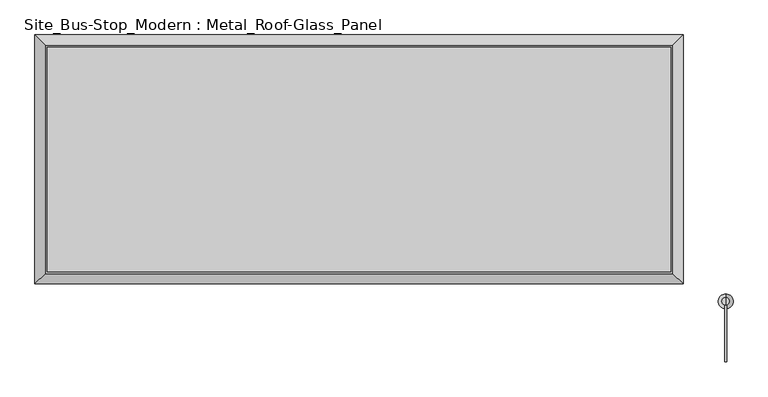
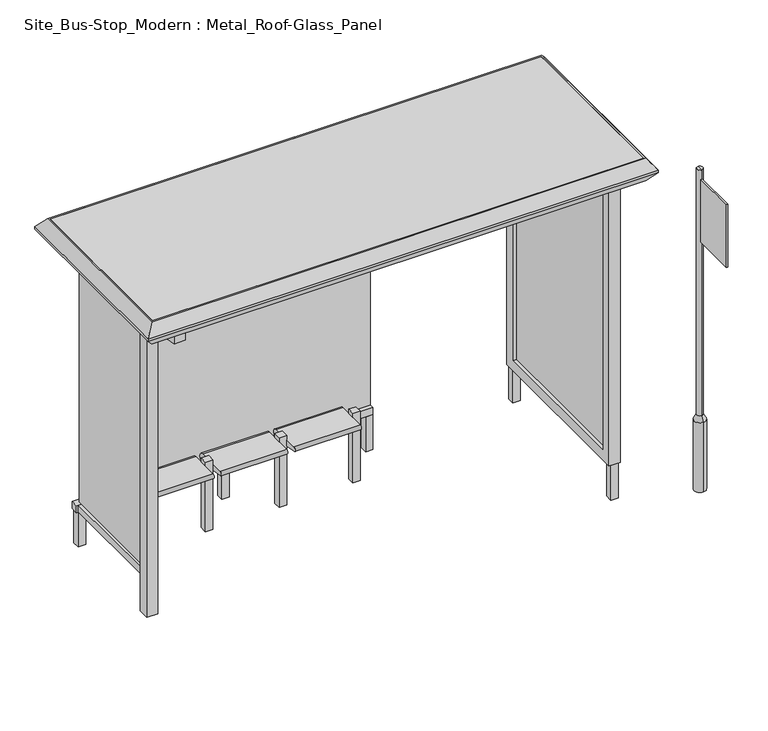
"""IFC4 building model written with IfcOpenShell, lengths in millimetres: geographic element geometry, Site_Bus-Stop_Modern : Metal_Roof-Glass_Panel."""

from ifc_helpers import new_model, si_unit, point, frame, frame_2d, origin, origin_with_axes, place, context, project, spatial, polyline, circle_curve, trimmed, segment, composite_curve, outline, extrude, faceted_brep, source, transform, mapped, element, save
from ifc_brep_helpers import plane_surface, cylinder_surface, revolved_surface, advanced_brep


def site_bus_stop_modern_metal_roof_glass_panel_3fdf870d(model_context):
    return source(origin(), model_context, "Body", "SolidModel", [
        extrude(outline(polyline([(1957.5, -1680.3732439), (1957.5, -1380.3732439), (1967.5, -1380.3732439), (1967.5, -1680.3732439), (1957.5, -1680.3732439)])), frame((0.0, 0.0, 1784.6), z_axis=(0.0, 0.0, 1.0), x_axis=(1.0, 0.0, 0.0)), (0.0, 0.0, 1.0), 450.0),
        advanced_brep(
        [(1962.5, -1398.2604073, 500.0), (1962.5, -1318.2604073, 500.0), (1962.5, -1318.2604073, 0.0), (1962.5, -1398.2604073, 0.0), (1962.5, -1378.2604073, 534.6), (1962.5, -1338.2604073, 534.6), (1962.5, -1378.2604073, 2300.0), (1962.5, -1338.2604073, 2300.0), (1962.5, -1358.2604073, 2300.0), (1962.5, -1358.2604073, 0.0)],
        [
            (0, 1, circle_curve(frame((1962.5, -1358.2604073, 500.0), z_axis=(0.0, 0.0, -1.0), x_axis=(0.0, 1.0, 0.0)), 40.0)),
            (1, 2),
            (2, 3, circle_curve(frame((1962.5, -1358.2604073, 0.0), z_axis=(0.0, 0.0, 1.0), x_axis=(0.0, 1.0, 0.0)), 40.0)),
            (3, 0),
            (1, 0, circle_curve(frame((1962.5, -1358.2604073, 500.0), z_axis=(0.0, 0.0, -1.0), x_axis=(0.0, 1.0, 0.0)), 40.0)),
            (3, 2, circle_curve(frame((1962.5, -1358.2604073, 0.0), z_axis=(0.0, 0.0, 1.0), x_axis=(0.0, 1.0, 0.0)), 40.0)),
            (4, 5, circle_curve(frame((1962.5, -1358.2604073, 534.6), z_axis=(0.0, 0.0, -1.0), x_axis=(0.0, 1.0, 0.0)), 20.0)),
            (5, 1),
            (0, 4),
            (5, 4, circle_curve(frame((1962.5, -1358.2604073, 534.6), z_axis=(0.0, 0.0, -1.0), x_axis=(0.0, 1.0, 0.0)), 20.0)),
            (6, 7, circle_curve(frame((1962.5, -1358.2604073, 2300.0), z_axis=(0.0, 0.0, -1.0), x_axis=(0.0, 1.0, 0.0)), 20.0)),
            (7, 5),
            (4, 6),
            (7, 6, circle_curve(frame((1962.5, -1358.2604073, 2300.0), z_axis=(0.0, 0.0, -1.0), x_axis=(0.0, 1.0, 0.0)), 20.0)),
            (8, 7),
            (6, 8),
            (2, 9),
            (9, 3),
        ],
        [
            cylinder_surface(frame((1962.5, -1358.2604073, -120.0), z_axis=(0.0, 0.0, 1.0), x_axis=(0.0, 1.0, 0.0)), 40.0),
            revolved_surface(polyline([(1962.5, -1318.2604073, 500.0), (1962.5, -1338.2604073, 534.6)]), (1962.5, -1358.2604073, -120.0), (0.0, 0.0, 1.0)),
            cylinder_surface(frame((1962.5, -1358.2604073, -120.0), z_axis=(0.0, 0.0, 1.0), x_axis=(0.0, 1.0, 0.0)), 20.0),
            plane_surface(frame((1962.5, -1358.2604073, 2300.0), z_axis=(0.0, 0.0, 1.0), x_axis=(0.0, 1.0, 0.0))),
            plane_surface(frame((1962.5, -1358.2604073, 0.0), z_axis=(0.0, 0.0, -1.0), x_axis=(0.0, 1.0, 0.0))),
        ],
        [
            (0, [[1, 2, 3, 4]]),
            (0, [[5, -4, 6, -2]]),
            (1, [[7, 8, -1, 9]]),
            (1, [[10, -9, -5, -8]]),
            (2, [[11, 12, -7, 13]]),
            (2, [[14, -13, -10, -12]]),
            (3, [[15, -11, 16]]),
            (3, [[-16, -14, -15]]),
            (4, [[-3, 17, 18]]),
            (4, [[-6, -18, -17]]),
        ],
    ),
        faceted_brep([(1735.0, 65.0, 2310.0), (1680.0, 10.0, 2380.0), (1680.0, -1210.0, 2380.0), (1735.0, -1265.0, 2310.0), (1735.0, 65.0, 2290.0), (1735.0, -1265.0, 2290.0), (1680.0, 10.0, 2220.0), (1680.0, -1210.0, 2220.0), (1670.0, 0.0, 2380.0), (1670.0, 0.0, 2220.0), (1670.0, -1200.0, 2220.0), (1670.0, -1200.0, 2380.0), (-1672.5, -1210.0, 2380.0), (-1727.5, -1265.0, 2310.0), (-1727.5, -1265.0, 2290.0), (-1672.5, -1210.0, 2220.0), (-1662.5, -1200.0, 2220.0), (-1662.5, -1200.0, 2380.0), (-1672.5, 10.0, 2380.0), (-1727.5, 65.0, 2310.0), (-1727.5, 65.0, 2290.0), (-1672.5, 10.0, 2220.0), (-1662.5, 0.0, 2220.0), (-1662.5, 0.0, 2380.0)], [[[0, 1, 2, 3]], [[4, 0, 3, 5]], [[6, 4, 5, 7]], [[8, 9, 10, 11]], [[3, 2, 12, 13]], [[5, 3, 13, 14]], [[7, 5, 14, 15]], [[11, 10, 16, 17]], [[13, 12, 18, 19]], [[14, 13, 19, 20]], [[15, 14, 20, 21]], [[17, 16, 22, 23]], [[19, 18, 1, 0]], [[20, 19, 0, 4]], [[21, 20, 4, 6]], [[7, 15, 21, 6], [9, 22, 16, 10]], [[23, 22, 9, 8]], [[1, 18, 12, 2], [11, 17, 23, 8]]]),
        extrude(outline(polyline([(-1662.5, -1200.0), (-1662.5, 0.0), (1670.0, 0.0), (1670.0, -1200.0), (-1662.5, -1200.0)])), frame((0.0, 0.0, 2220.0), z_axis=(0.0, 0.0, 1.0), x_axis=(1.0, 0.0, 0.0)), (0.0, 0.0, 1.0), 160.0),
        extrude(outline(polyline([(1490.0, -50.0), (1490.0, -1150.0), (1480.0, -1150.0), (1480.0, -50.0), (1490.0, -50.0)])), frame((0.0, 0.0, 300.0), z_axis=(0.0, 0.0, 1.0), x_axis=(1.0, 0.0, 0.0)), (0.0, 0.0, 1.0), 1870.0),
        extrude(outline(polyline([(1460.0, -1150.0), (1460.0, -50.0), (1470.0, -50.0), (1470.0, -1150.0), (1460.0, -1150.0)])), frame((0.0, 0.0, 300.0), z_axis=(0.0, 0.0, 1.0), x_axis=(1.0, 0.0, 0.0)), (0.0, 0.0, 1.0), 1870.0),
        faceted_brep([(1512.5, 0.0, 250.0), (1437.5, 0.0, 250.0), (1437.5, 0.0, 2220.0), (1512.5, 0.0, 2220.0), (1487.5, -75.0, 325.0), (1512.5, -75.0, 325.0), (1512.5, -75.0, 2145.0), (1487.5, -75.0, 2145.0), (1462.5, -50.0, 300.0), (1487.5, -50.0, 300.0), (1487.5, -50.0, 2170.0), (1462.5, -50.0, 2170.0), (1437.5, -75.0, 325.0), (1462.5, -75.0, 325.0), (1462.5, -75.0, 2145.0), (1437.5, -75.0, 2145.0), (1437.5, -1200.0, 2220.0), (1512.5, -1200.0, 2220.0), (1512.5, -1125.0, 2145.0), (1487.5, -1125.0, 2145.0), (1487.5, -1150.0, 2170.0), (1462.5, -1150.0, 2170.0), (1462.5, -1125.0, 2145.0), (1437.5, -1125.0, 2145.0), (1437.5, -1200.0, 250.0), (1512.5, -1200.0, 250.0), (1512.5, -1125.0, 325.0), (1487.5, -1125.0, 325.0), (1487.5, -1150.0, 300.0), (1462.5, -1150.0, 300.0), (1462.5, -1125.0, 325.0), (1437.5, -1125.0, 325.0)], [[[0, 1, 2, 3]], [[4, 5, 6, 7]], [[8, 9, 10, 11]], [[12, 13, 14, 15]], [[3, 2, 16, 17]], [[7, 6, 18, 19]], [[11, 10, 20, 21]], [[15, 14, 22, 23]], [[17, 16, 24, 25]], [[19, 18, 26, 27]], [[21, 20, 28, 29]], [[23, 22, 30, 31]], [[25, 24, 1, 0]], [[3, 17, 25, 0], [5, 26, 18, 6]], [[27, 26, 5, 4]], [[9, 28, 20, 10], [7, 19, 27, 4]], [[29, 28, 9, 8]], [[11, 21, 29, 8], [13, 30, 22, 14]], [[31, 30, 13, 12]], [[1, 24, 16, 2], [15, 23, 31, 12]]]),
        extrude(outline(polyline([(500.0, -20.0), (-1470.0, -20.0), (-1470.0, -10.0), (500.0, -10.0), (500.0, -20.0)])), frame((0.0, 0.0, 300.0), z_axis=(0.0, 0.0, 1.0), x_axis=(1.0, 0.0, 0.0)), (0.0, 0.0, 1.0), 1920.0),
        extrude(outline(polyline([(-800.0, 300.0), (-800.0, 2100.0), (-25.0, 2158.125), (-25.0, 300.0), (-800.0, 300.0)])), frame((-1480.0, 0.0, 0.0), z_axis=(1.0, 0.0, 0.0), x_axis=(0.0, 1.0, 0.0)), (0.0, 0.0, 1.0), 10.0),
        extrude(outline(composite_curve([segment(trimmed(circle_curve(frame_2d((-171.5367578, 436.9988667)), 33.0011333), [point((-171.5367578, 470.0))], [point((-171.5367578, 403.9977334))], False, "CARTESIAN"), True, "CONTINUOUS"), segment(polyline([(-171.5367578, 403.9977334), (-376.5367578, 440.1447644)]), True, "CONTINUOUS"), segment(trimmed(circle_curve(frame_2d((-376.5367578, 455.0723822)), 14.9276178), [point((-376.5367578, 440.1447644))], [point((-376.5367578, 470.0))], False, "CARTESIAN"), True, "CONTINUOUS"), segment(polyline([(-376.5367578, 470.0), (-171.5367578, 470.0)]), True, "CONTINUOUS")], self_intersect=False)), frame((-225.0, 0.0, 0.0), z_axis=(1.0, 0.0, 0.0), x_axis=(0.0, 1.0, 0.0)), (0.0, 0.0, 1.0), 450.0),
        extrude(outline(composite_curve([segment(trimmed(circle_curve(frame_2d((-171.5367578, 436.9988667)), 33.0011333), [point((-171.5367578, 470.0))], [point((-171.5367578, 403.9977334))], False, "CARTESIAN"), True, "CONTINUOUS"), segment(polyline([(-171.5367578, 403.9977334), (-376.5367578, 440.1447644)]), True, "CONTINUOUS"), segment(trimmed(circle_curve(frame_2d((-376.5367578, 455.0723822)), 14.9276178), [point((-376.5367578, 440.1447644))], [point((-376.5367578, 470.0))], False, "CARTESIAN"), True, "CONTINUOUS"), segment(polyline([(-376.5367578, 470.0), (-171.5367578, 470.0)]), True, "CONTINUOUS")], self_intersect=False)), frame((-725.0, 0.0, 0.0), z_axis=(1.0, 0.0, 0.0), x_axis=(0.0, 1.0, 0.0)), (0.0, 0.0, 1.0), 450.0),
        extrude(outline(composite_curve([segment(trimmed(circle_curve(frame_2d((-173.0011333, 436.9988667)), 33.0011333), [point((-173.0011333, 470.0))], [point((-173.0011333, 403.9977334))], False, "CARTESIAN"), True, "CONTINUOUS"), segment(polyline([(-173.0011333, 403.9977334), (-378.0011333, 440.1447644)]), True, "CONTINUOUS"), segment(trimmed(circle_curve(frame_2d((-378.0011333, 455.0723822)), 14.9276178), [point((-378.0011333, 440.1447644))], [point((-378.0011333, 470.0))], False, "CARTESIAN"), True, "CONTINUOUS"), segment(polyline([(-378.0011333, 470.0), (-173.0011333, 470.0)]), True, "CONTINUOUS")], self_intersect=False)), frame((-1225.0, 0.0, 0.0), z_axis=(1.0, 0.0, 0.0), x_axis=(0.0, 1.0, 0.0)), (0.0, 0.0, 1.0), 450.0),
        extrude(outline(polyline([(-1200.0, 2220.0), (0.0, 2220.0), (0.0, 2160.0), (-800.0, 2100.0), (-875.0, 2100.0), (-1200.0, 2160.0), (-1200.0, 2220.0)])), frame((-1512.5, 0.0, 0.0), z_axis=(1.0, 0.0, 0.0), x_axis=(0.0, 1.0, 0.0)), (0.0, 0.0, 1.0), 75.0),
        extrude(outline(polyline([(-1437.5, -800.0), (-1437.5, -875.0), (-1512.5, -875.0), (-1512.5, -800.0), (-1437.5, -800.0)])), origin_with_axes(), (0.0, 0.0, 1.0), 2100.0),
        extrude(outline(polyline([(-1500.0, -50.0), (-1450.0, -50.0), (-1450.0, -800.0), (-1500.0, -800.0), (-1500.0, -50.0)])), frame((0.0, 0.0, 250.0), z_axis=(0.0, 0.0, 1.0), x_axis=(1.0, 0.0, 0.0)), (0.0, 0.0, 1.0), 50.0),
        extrude(outline(polyline([(500.0, 0.0), (500.0, -50.0), (-1512.5, -50.0), (-1512.5, 0.0), (500.0, 0.0)])), frame((0.0, 0.0, 250.0), z_axis=(0.0, 0.0, 1.0), x_axis=(1.0, 0.0, 0.0)), (0.0, 0.0, 1.0), 50.0),
        extrude(outline(polyline([(275.0, -240.0), (275.0, -290.0), (225.0, -290.0), (225.0, -240.0), (275.0, -240.0)])), origin_with_axes(), (0.0, 0.0, 1.0), 500.0),
        extrude(outline(polyline([(-225.0, -240.0), (-225.0, -290.0), (-275.0, -290.0), (-275.0, -240.0), (-225.0, -240.0)])), origin_with_axes(), (0.0, 0.0, 1.0), 500.0),
        extrude(outline(polyline([(-725.0, -240.0), (-725.0, -290.0), (-775.0, -290.0), (-775.0, -240.0), (-725.0, -240.0)])), origin_with_axes(), (0.0, 0.0, 1.0), 500.0),
        extrude(outline(polyline([(-1225.0, -240.0), (-1225.0, -290.0), (-1275.0, -290.0), (-1275.0, -240.0), (-1225.0, -240.0)])), origin_with_axes(), (0.0, 0.0, 1.0), 500.0),
        extrude(outline(polyline([(1500.0, -1150.0), (1500.0, -1200.0), (1450.0, -1200.0), (1450.0, -1150.0), (1500.0, -1150.0)])), origin_with_axes(), (0.0, 0.0, 1.0), 250.0),
        extrude(outline(polyline([(1500.0, 0.0), (1500.0, -50.0), (1450.0, -50.0), (1450.0, 0.0), (1500.0, 0.0)])), origin_with_axes(), (0.0, 0.0, 1.0), 250.0),
        extrude(outline(polyline([(500.0, 0.0), (500.0, -50.0), (450.0, -50.0), (450.0, 0.0), (500.0, 0.0)])), origin_with_axes(), (0.0, 0.0, 1.0), 250.0),
        extrude(outline(polyline([(-475.0, 0.0), (-475.0, -50.0), (-525.0, -50.0), (-525.0, 0.0), (-475.0, 0.0)])), origin_with_axes(), (0.0, 0.0, 1.0), 250.0),
        extrude(outline(polyline([(-1450.0, 0.0), (-1450.0, -50.0), (-1500.0, -50.0), (-1500.0, 0.0), (-1450.0, 0.0)])), origin_with_axes(), (0.0, 0.0, 1.0), 250.0),
    ])


if __name__ == "__main__":
    model = new_model("IFC4")
    model_context = context("Model", 3, world=origin())
    ifc_project = project(units=[si_unit("LENGTHUNIT", "METRE", prefix="MILLI")], contexts=[model_context])
    site = spatial("IfcSite", under=ifc_project)
    building = spatial("IfcBuilding", under=site)
    placement = place(None, origin())
    site_bus_stop_modern_metal_roof_glass_panel_shape = site_bus_stop_modern_metal_roof_glass_panel_3fdf870d(model_context)
    element("IfcGeographicElement", 1, ObjectType="Site_Bus-Stop_Modern : Metal_Roof-Glass_Panel", at=placement, inside=building, context=model_context, shape_type="MappedRepresentation", body=[
        mapped(site_bus_stop_modern_metal_roof_glass_panel_shape, transform((0.0, 0.0, 0.0), x_axis=(1.0, 0.0, 0.0), y_axis=(0.0, 1.0, 0.0), z_axis=(0.0, 0.0, 1.0))),
    ])
    save(model, "model.ifc")

# Revit data of these elements
# Type "Site_Bus-Stop_Modern : Metal_Roof-Glass_Panel"
#   Material Structure = Metal - Aluminium Satin Hammered
#   Material Seat = Plastic - Red Light Textured
#   Material Roof = Metal - Aluminium Satin
#   Material Bus Stop Sign = Plastic - White Smooth
#   Material Bus Stop Post = Paint - Grey Medium
#   Material Glass = Glass - Blue Dark
# Element 1 (IfcGeographicElement, "Site_Bus-Stop_Modern : Metal_Roof-Glass_Panel")
#   Materials on its faces: "Metal - Aluminium Satin Hammered", "Glass - Blue Dark", "Metal - Aluminium Satin", "Plastic - Red Light Textured", "Paint - Grey Medium", "Plastic - White Smooth"
# Materials
#   "Metal - Aluminium Satin Hammered": class "Metal", colour RGB 247 247 247, transparency 0
#   "Plastic - Red Light Textured": class "Plastic", colour RGB 247 135 0, transparency 0
#   "Metal - Aluminium Satin": class "Metal", colour RGB 247 247 247, transparency 0
#   "Plastic - White Smooth": class "Plastic", colour RGB 249 249 249, transparency 0
#   "Paint - Grey Medium": class "Paint", colour RGB 162 162 162, transparency 0
#   "Glass - Blue Dark": class "Glass", colour RGB 57 95 150, transparency 0.7
